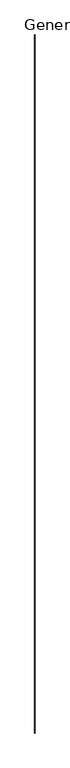
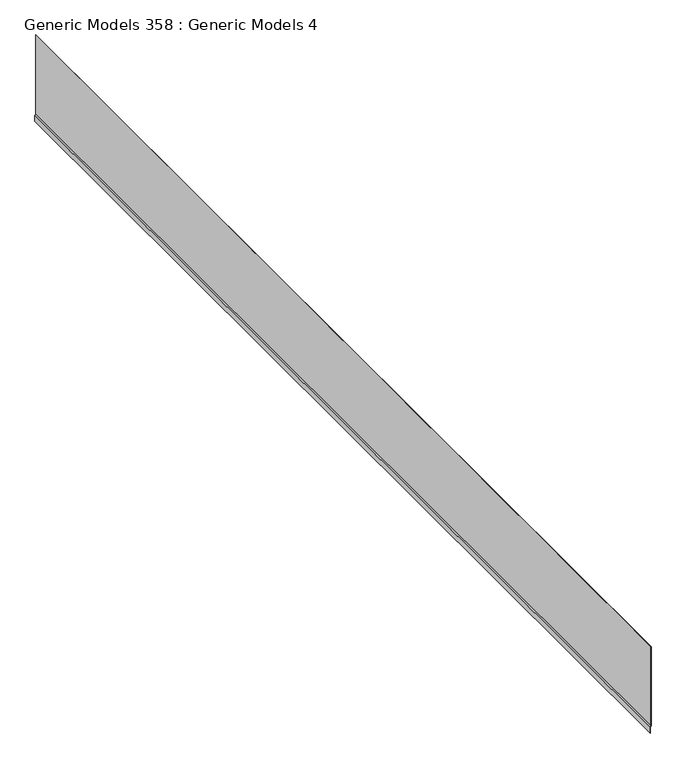
"""IFC4 building model written with IfcOpenShell, lengths in millimetres: proxy geometry, Generic Models 358 : Generic Models 4."""

from ifc_helpers import new_model, si_unit, frame, origin, place, context, project, spatial, polyline, outline, extrude, source, transform, mapped, element, save


def generic_models_358_generic_models_4_c9dea4d0(model_context):
    return source(origin(), model_context, "Body", "SweptSolid", [
        extrude(outline(polyline([(126737.3262036, -6624.0173796), (127239.1064906, -6624.0173796), (127239.1064906, -6624.8111296), (126737.4661632, -6624.8111296), (126726.3724169, -6628.848923), (126693.0624044, -6628.848923), (126693.0624044, -6628.055173), (126726.2324574, -6628.055173), (126737.3262036, -6624.0173796)])), frame((0.0, -6864.9230338, 0.0), z_axis=(0.0, 1.0, 0.0), x_axis=(0.0, 0.0, 1.0)), (0.0, 0.0, 1.0), 6400.8),
    ])


if __name__ == "__main__":
    model = new_model("IFC4")
    model_context = context("Model", 3, world=origin())
    ifc_project = project(units=[si_unit("LENGTHUNIT", "METRE", prefix="MILLI")], contexts=[model_context])
    site = spatial("IfcSite", under=ifc_project)
    building = spatial("IfcBuilding", under=site)
    placement = place(None, origin())
    generic_models_358_generic_models_4_shape = generic_models_358_generic_models_4_c9dea4d0(model_context)
    element("IfcBuildingElementProxy", 1, Name="Generic Models 358 : Generic Models 4", ObjectType="Generic Models 358 : Generic Models 4", at=placement, inside=building, context=model_context, shape_type="MappedRepresentation", body=[
        mapped(generic_models_358_generic_models_4_shape, transform((0.0, 0.0, 0.0), x_axis=(1.0, 0.0, 0.0), y_axis=(0.0, 1.0, 0.0), z_axis=(0.0, 0.0, 1.0))),
    ])
    save(model, "model.ifc")

# Revit data of these elements
# Element 1 (IfcBuildingElementProxy, "Generic Models 358 : Generic Models 4")
#   Materials on its faces: "_(2) LAYERS NO. 30 ASTM D226 ASPHALT SATURATED ORGANIC FELT"
# Materials
#   "_(2) LAYERS NO. 30 ASTM D226 ASPHALT SATURATED ORGANIC FELT": class "Generic", colour RGB 67 154 161, transparency 0, Cost = 0
